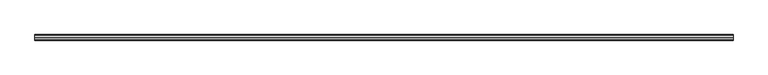
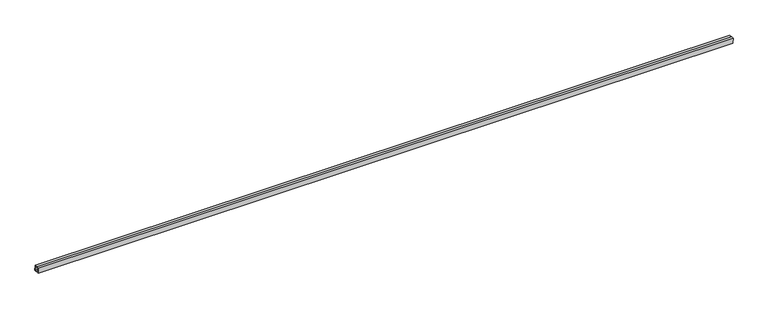
"""IFC4 building model written with IfcOpenShell, lengths in millimetres: proxy geometry, Inner panel:Inner panel:1:Inner panel:1 : Inner panel:Inner panel:300324:2:Inner panel:1:Inner panel:1 : Inner panel:Inner panel:300324:2 : Inner panel:Inner panel:1:Inner panel:1 : Inner panel:Inner panel:300324:300043:44 : Inner panel:Inner panel:1:Inner panel:1 : Inner panel:Inner panel:300324:2:Inner panel:1:Inner panel:1 : Inner panel:Inner panel:300324:2 : Inner panel:Inner panel:1:Inner panel:1 : Inner panel:Inner panel:300324:300043:308120."""

import ifcopenshell
import ifcopenshell.guid

model = None  # the IFC model being written
_history = None  # IfcOwnerHistory: only IFC2X3 demands one
_inside = {}  # id of a spatial element -> (the spatial element, [elements in it])
_under = {}  # id of a project, library or spatial element -> (it, [spatial elements below it])
_declared = {}  # id of a project -> (the project, [libraries it declares])
_typed = {}  # id of a type object -> (the type object, [elements of that type])
_made_of = {}  # id of a material, layer set ... -> (it, [elements and type objects made of it])


def new_model(schema):
    """Start an empty IFC model of exactly this schema.

    Asked for "IFC4X3", IfcOpenShell would pick the latest addendum, in which some entities
    have other attributes; the version numbers below select the first issue.
    IFC2X3 requires an IfcOwnerHistory on every rooted entity: one is made here for all.
    """
    global model, _history
    if schema == "IFC4X3":
        model = ifcopenshell.file(schema_version=(4, 3, 0, 0))
    else:
        model = ifcopenshell.file(schema=schema)
    _inside.clear()
    _under.clear()
    _declared.clear()
    _typed.clear()
    _made_of.clear()
    _history = None
    if model.schema == "IFC2X3":
        org = make("IfcOrganization", Name="unknown")
        user = make(
            "IfcPersonAndOrganization",
            ThePerson=make("IfcPerson", FamilyName="unknown"),
            TheOrganization=org,
        )
        app = make(
            "IfcApplication",
            ApplicationDeveloper=org,
            Version="unknown",
            ApplicationFullName="unknown",
            ApplicationIdentifier="unknown",
        )
        _history = make(
            "IfcOwnerHistory",
            OwningUser=user,
            OwningApplication=app,
            ChangeAction="ADDED",
            CreationDate=0,
        )
    return model


def make(cls, **values):
    """One entity of the class cls with the attributes given. An attribute that is None is left unset."""
    return model.create_entity(
        cls, **{name: value for name, value in values.items() if value is not None}
    )


def rooted(cls, **values):
    """An entity with a GlobalId (a new one), such as an element, a storey or a relation."""
    return make(cls, GlobalId=ifcopenshell.guid.new(), OwnerHistory=_history, **values)


def si_unit(unit_type, name, prefix=None):
    """IfcSIUnit, for example si_unit("LENGTHUNIT", "METRE", prefix="MILLI")."""
    return make("IfcSIUnit", UnitType=unit_type, Prefix=prefix, Name=name)


def assignment(units):
    """IfcUnitAssignment: the units of a project."""
    return None if units is None else make("IfcUnitAssignment", Units=units)


def point(xyz):
    """IfcCartesianPoint."""
    return None if xyz is None else make("IfcCartesianPoint", Coordinates=xyz)


def direction(xyz):
    """IfcDirection."""
    return None if xyz is None else make("IfcDirection", DirectionRatios=xyz)


def frame(location, z_axis=None, x_axis=None):
    """IfcAxis2Placement3D, a coordinate frame: its origin and axes. An axis left out is left unset."""
    return make(
        "IfcAxis2Placement3D",
        Location=point(location),
        Axis=direction(z_axis),
        RefDirection=direction(x_axis),
    )


def origin():
    """The frame at (0, 0, 0) with its axes left unset."""
    return frame((0.0, 0.0, 0.0))


def place(relative_to, where):
    """IfcLocalPlacement: puts the frame where relative to a parent placement (None: the world)."""
    return make(
        "IfcLocalPlacement", PlacementRelTo=relative_to, RelativePlacement=where
    )


def context(
    kind, dimensions, precision=None, world=None, true_north=None, identifier=None
):
    """IfcGeometricRepresentationContext, for example the 3D "Model" context."""
    return make(
        "IfcGeometricRepresentationContext",
        ContextIdentifier=identifier,
        ContextType=kind,
        CoordinateSpaceDimension=dimensions,
        Precision=precision,
        WorldCoordinateSystem=world,
        TrueNorth=true_north,
    )


def project(units=None, contexts=None):
    """IfcProject with its units and contexts."""
    return rooted(
        "IfcProject",
        Name="project",
        RepresentationContexts=contexts,
        UnitsInContext=assignment(units),
    )


def spatial(cls, under=None, at=None, **own):
    """A site, building, storey or space (cls), placed at a placement, below another one or the project."""
    s = rooted(cls, ObjectPlacement=at, **own)
    if under is not None:
        _under.setdefault(under.id(), (under, []))[1].append(s)
    return s


def polyline(points):
    """IfcPolyline through the points."""
    return make("IfcPolyline", Points=[point(p) for p in points])


def outline(outer, holes=None, kind="AREA"):
    """IfcArbitraryClosedProfileDef: a profile drawn as a closed curve; with holes, ...WithVoids."""
    if holes is None:
        return make("IfcArbitraryClosedProfileDef", ProfileType=kind, OuterCurve=outer)
    return make(
        "IfcArbitraryProfileDefWithVoids",
        ProfileType=kind,
        OuterCurve=outer,
        InnerCurves=holes,
    )


def extrude(swept, where, along, depth):
    """IfcExtrudedAreaSolid: the profile swept, set in the frame where, extruded along a direction by depth."""
    return make(
        "IfcExtrudedAreaSolid",
        SweptArea=swept,
        Position=where,
        ExtrudedDirection=direction(along),
        Depth=depth,
    )


def shape(context_of_items, identifier, shape_type, items):
    """IfcShapeRepresentation: the items that make up one representation, for example the "Body"."""
    return make(
        "IfcShapeRepresentation",
        ContextOfItems=context_of_items,
        RepresentationIdentifier=identifier,
        RepresentationType=shape_type,
        Items=items,
    )


def source(mapping_origin, context_of_items, identifier, shape_type, items):
    """IfcRepresentationMap: a shape defined once, which mapped items show again and again."""
    return make(
        "IfcRepresentationMap",
        MappingOrigin=mapping_origin,
        MappedRepresentation=shape(context_of_items, identifier, shape_type, items),
    )


def transform(
    local_origin,
    x_axis=None,
    y_axis=None,
    z_axis=None,
    scale=None,
    scale2=None,
    scale3=None,
    uniform=True,
):
    """IfcCartesianTransformationOperator3D, or its non-uniform kind. x_axis, y_axis, z_axis: its Axis1, 2, 3."""
    if uniform:
        return make(
            "IfcCartesianTransformationOperator3D",
            Axis1=direction(x_axis),
            Axis2=direction(y_axis),
            LocalOrigin=point(local_origin),
            Scale=scale,
            Axis3=direction(z_axis),
        )
    return make(
        "IfcCartesianTransformationOperator3DnonUniform",
        Axis1=direction(x_axis),
        Axis2=direction(y_axis),
        LocalOrigin=point(local_origin),
        Scale=scale,
        Axis3=direction(z_axis),
        Scale2=scale2,
        Scale3=scale3,
    )


def mapped(mapping_source, mapping_target):
    """IfcMappedItem: shows the shape of a source again, moved by a transform."""
    return make(
        "IfcMappedItem", MappingSource=mapping_source, MappingTarget=mapping_target
    )


def made_of(thing, what):
    """Note that an element or type object is made of a material, layer set ...; save() writes the relation."""
    if what is not None:
        _made_of.setdefault(what.id(), (what, []))[1].append(thing)
    return thing


def element(
    cls,
    number,
    at=None,
    inside=None,
    cuts=None,
    type_object=None,
    material=None,
    context=None,
    identifier="Body",
    shape_type=None,
    held_by="IfcProductDefinitionShape",
    body=None,
    shapes=None,
    **own,
):
    """One element of the class cls, such as IfcWall. Its Tag is "e" and its number.

    at: its placement. inside: the storey or other place that contains it. cuts: it is an
    opening in that element (IfcRelVoidsElement). A single representation is given by context,
    identifier, shape_type and body (its items); several are given by shapes. held_by: the class
    of the entity that holds the representations. save() writes the other relations.
    """
    e = rooted(cls, Tag="e%d" % number, ObjectPlacement=at, **own)
    if body is not None:
        shapes = [shape(context, identifier, shape_type, body)]
    if shapes is not None:
        e.Representation = make(held_by, Representations=shapes)
    if inside is not None:
        _inside.setdefault(inside.id(), (inside, []))[1].append(e)
    if cuts is not None:
        rooted(
            "IfcRelVoidsElement", RelatingBuildingElement=cuts, RelatedOpeningElement=e
        )
    if type_object is not None:
        _typed.setdefault(type_object.id(), (type_object, []))[1].append(e)
    return made_of(e, material)


def aggregate(whole, parts):
    """IfcRelAggregates: a whole, such as a stair, and the parts it consists of."""
    return rooted("IfcRelAggregates", RelatingObject=whole, RelatedObjects=parts)


def save(model, path):
    """Write the relations noted so far, then the file.

    IfcRelAggregates (storeys below a building ...), IfcRelContainedInSpatialStructure (elements
    in a storey), IfcRelDefinesByType, IfcRelAssociatesMaterial and IfcRelDeclares: one each for
    every whole, place, type object, material and project.
    """
    for whole, parts in _under.values():
        aggregate(whole, parts)
    for where, things in _inside.values():
        rooted(
            "IfcRelContainedInSpatialStructure",
            RelatedElements=things,
            RelatingStructure=where,
        )
    for kind, things in _typed.values():
        rooted("IfcRelDefinesByType", RelatedObjects=things, RelatingType=kind)
    for what, things in _made_of.values():
        rooted("IfcRelAssociatesMaterial", RelatedObjects=things, RelatingMaterial=what)
    for by, libraries in _declared.values():
        rooted("IfcRelDeclares", RelatingContext=by, RelatedDefinitions=libraries)
    model.write(path)


def generic_models_5d710027(model_context):
    return source(origin(), model_context, "Body", "SweptSolid", [
        extrude(outline(polyline([(-581211.0091179, 3857.8017792), (-581192.7686948, 3858.5617968), (-581191.182571, 3820.4948267), (-581229.2495411, 3818.908703), (-581230.8356649, 3856.9756731), (-581212.5952417, 3857.7356907), (-581212.496109, 3855.3565051), (-581228.3573465, 3854.6956202), (-581226.9694882, 3821.3870213), (-581193.6608894, 3822.7748796), (-581195.0487477, 3856.0834785), (-581210.9099852, 3855.4225936), (-581211.0091179, 3857.8017792)])), frame((607854.1367239, 0.0, 0.0), z_axis=(1.0, 0.0, 0.0), x_axis=(0.0, 1.0, 0.0)), (0.0, 0.0, 1.0), 4876.8),
    ])


if __name__ == "__main__":
    model = new_model("IFC4")
    model_context = context("Model", 3, world=origin())
    ifc_project = project(units=[si_unit("LENGTHUNIT", "METRE", prefix="MILLI")], contexts=[model_context])
    site = spatial("IfcSite", under=ifc_project)
    building = spatial("IfcBuilding", under=site)
    placement = place(None, origin())
    generic_models_shape = generic_models_5d710027(model_context)
    element("IfcBuildingElementProxy", 1, Name="Inner panel:Inner panel:1:Inner panel:1 : Inner panel:Inner panel:300324:2:Inner panel:1:Inner panel:1 : Inner panel:Inner panel:300324:2 : Inner panel:Inner panel:1:Inner panel:1 : Inner panel:Inner panel:300324:300043:44 : Inner panel:Inner panel:1:Inner panel:1 : Inner panel:Inner panel:300324:2:Inner panel:1:Inner panel:1 : Inner panel:Inner panel:300324:2 : Inner panel:Inner panel:1:Inner panel:1 : Inner panel:Inner panel:300324:300043:308120", ObjectType="Inner panel:Inner panel:1:Inner panel:1 : Inner panel:Inner panel:300324:2:Inner panel:1:Inner panel:1 : Inner panel:Inner panel:300324:2 : Inner panel:Inner panel:1:Inner panel:1 : Inner panel:Inner panel:300324:300043:44 : Inner panel:Inner panel:1:Inner panel:1 : Inner panel:Inner panel:300324:2:Inner panel:1:Inner panel:1 : Inner panel:Inner panel:300324:2 : Inner panel:Inner panel:1:Inner panel:1 : Inner panel:Inner panel:300324:300043:308120", at=placement, inside=building, context=model_context, shape_type="MappedRepresentation", body=[
        mapped(generic_models_shape, transform((0.0, 0.0, 0.0), x_axis=(1.0, 0.0, 0.0), y_axis=(0.0, 1.0, 0.0), z_axis=(0.0, 0.0, 1.0))),
    ])
    save(model, "model.ifc")

# Revit data of these elements
# Type "Inner panel:Inner panel:1:Inner panel:1 : Inner panel:Inner panel:300324:2:Inner panel:1:Inner panel:1 : Inner panel:Inner panel:300324:2 : Inner panel:Inner panel:1:Inner panel:1 : Inner panel:Inner panel:300324:300043:44 : Inner panel:Inner panel:1:Inner panel:1 : Inner panel:Inner panel:300324:2:Inner panel:1:Inner panel:1 : Inner panel:Inner panel:300324:2 : Inner panel:Inner panel:1:Inner panel:1 : Inner panel:Inner panel:300324:300043:308120"
#   NameOverride = "Inner panel:Inner panel:1:Inner panel:1 : Inner panel:Inner panel:300324:2:Inner panel:1:Inner panel:1 : Inner panel:Inner panel:300324:2 : Inner panel:Inner panel:1:Inner panel:1 : Inner panel:Inner panel:300324:300043:308120"
#   ObjectTypeOverride = "Inner panel:1:Inner panel:1 : Inner panel:Inner panel:300324:2 : Inner panel:Inner panel:1:Inner panel:1 : Inner panel:Inner panel:300324:300043"
#   Reference = "Inner panel"
#   Tag = "308120"
# Element 1 (IfcBuildingElementProxy, "Inner panel:Inner panel:1:Inner panel:1 : Inner panel:Inner panel:300324:2:Inner panel:1:Inner panel:1 : Inner panel:Inner panel:300324:2 : Inner panel:Inner panel:1:Inner panel:1 : Inner panel:Inner panel:300324:300043:44 : Inner panel:Inner panel:1:Inner panel:1 : Inner panel:Inner panel:300324:2:Inner panel:1:Inner panel:1 : Inner panel:Inner panel:300324:2 : Inner panel:Inner panel:1:Inner panel:1 : Inner panel:Inner panel:300324:300043:308120")
#   Materials on its faces: "1 1/2\" X 1 1/2\" SPLIT-SEAM SQUARE TUBING (~24\" CANTILEVER FROM C.L. OF GLULAM)"
# Materials
#   "1 1/2\" X 1 1/2\" SPLIT-SEAM SQUARE TUBING (~24\" CANTILEVER FROM C.L. OF GLULAM)": class "Unassigned", colour RGB 202 201 200, transparency 0, Cost = 0
